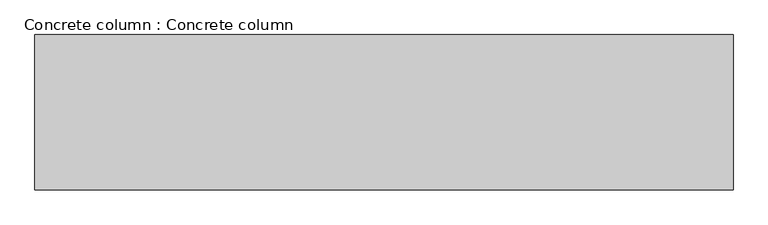
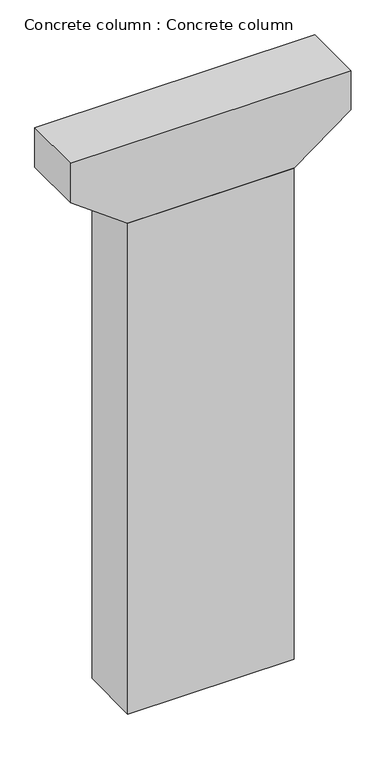
"""IFC4 building model written with IfcOpenShell, lengths in millimetres: proxy geometry, Concrete column : Concrete column."""

from ifc_helpers import new_model, si_unit, frame, origin, origin_with_axes, place, context, project, spatial, polyline, outline, extrude, source, transform, mapped, element, save


def concrete_column_concrete_column_f1e0fce3(model_context):
    return source(origin(), model_context, "Body", "SweptSolid", [
        extrude(outline(polyline([(29000.0, 6750.0), (29000.0, -6750.0), (27000.0, -6750.0), (25000.0, -4000.0), (25000.0, 4000.0), (27000.0, 6750.0), (29000.0, 6750.0)])), frame((0.0, -1500.0, 0.0), z_axis=(0.0, 1.0, 0.0), x_axis=(0.0, 0.0, 1.0)), (0.0, 0.0, 1.0), 3000.0),
        extrude(outline(polyline([(4000.0, 1500.0), (4000.0, -1500.0), (-4000.0, -1500.0), (-4000.0, 1500.0), (4000.0, 1500.0)])), origin_with_axes(), (0.0, 0.0, 1.0), 25000.0),
    ])


if __name__ == "__main__":
    model = new_model("IFC4")
    model_context = context("Model", 3, world=origin())
    ifc_project = project(units=[si_unit("LENGTHUNIT", "METRE", prefix="MILLI")], contexts=[model_context])
    site = spatial("IfcSite", under=ifc_project)
    building = spatial("IfcBuilding", under=site)
    placement = place(None, origin())
    concrete_column_concrete_column_shape = concrete_column_concrete_column_f1e0fce3(model_context)
    element("IfcBuildingElementProxy", 1, Name="Concrete column : Concrete column", ObjectType="Concrete column : Concrete column", at=placement, inside=building, context=model_context, shape_type="MappedRepresentation", body=[
        mapped(concrete_column_concrete_column_shape, transform((0.0, 0.0, 0.0), x_axis=(1.0, 0.0, 0.0), y_axis=(0.0, 1.0, 0.0), z_axis=(0.0, 0.0, 1.0))),
    ])
    save(model, "model.ifc")

# Revit data of these elements
# Type "Concrete column : Concrete column"
#   Height = 25000 mm
#   Bottom width [instance default] = 3000 mm
#   Bottom length [instance default] = 8000 mm
#   Default Elevation = 0
